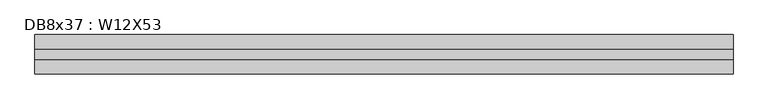
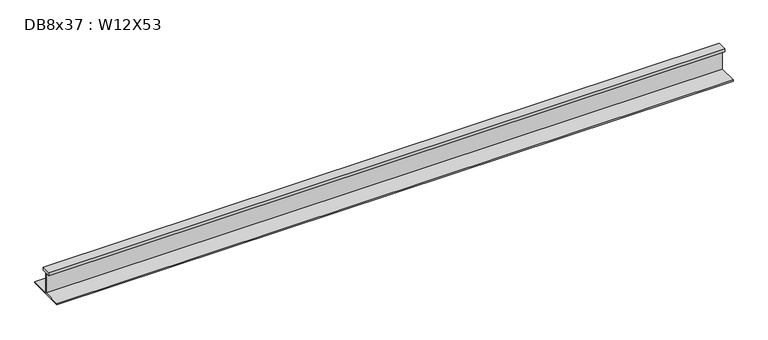
"""IFC4 building model written with IfcOpenShell, lengths in millimetres: beam geometry, DB8x37 : W12X53."""

from ifc_helpers import new_model, si_unit, frame, origin, place, context, project, spatial, polyline, outline, extrude, source, transform, mapped, element, save


def db8x37_w12x53_95cbac0b(model_context):
    return source(origin(), model_context, "Body", "SweptSolid", [
        extrude(outline(polyline([(38.1, 145.415), (38.1, 120.015), (2.921, 120.015), (2.921, -48.4505), (152.4, -48.4505), (152.4, -58.1025), (-152.4, -58.1025), (-152.4, -48.4505), (-2.921, -48.4505), (-2.921, 120.015), (-38.1, 120.015), (-38.1, 145.415), (38.1, 145.415)])), frame((-2691.1319305, 0.0, 0.0), z_axis=(1.0, 0.0, 0.0), x_axis=(0.0, 1.0, 0.0)), (0.0, 0.0, 1.0), 5387.0585186),
    ])


if __name__ == "__main__":
    model = new_model("IFC4")
    model_context = context("Model", 3, world=origin())
    ifc_project = project(units=[si_unit("LENGTHUNIT", "METRE", prefix="MILLI")], contexts=[model_context])
    site = spatial("IfcSite", under=ifc_project)
    building = spatial("IfcBuilding", under=site)
    placement = place(None, origin())
    db8x37_w12x53_shape = db8x37_w12x53_95cbac0b(model_context)
    element("IfcBeam", 1, ObjectType="DB8x37 : W12X53", at=placement, inside=building, context=model_context, shape_type="MappedRepresentation", body=[
        mapped(db8x37_w12x53_shape, transform((0.0, 0.0, 0.0), x_axis=(1.0, 0.0, 0.0), y_axis=(0.0, 1.0, 0.0), z_axis=(0.0, 0.0, 1.0))),
    ])
    save(model, "model.ifc")

# Revit data of these elements
# Type "DB8x37 : W12X53"
#   Assembly Code = "B10"
#   W = 53
#   Length [instance default] = 5' - 0"
#   bf = 0' - 10"
#   d = 1' - 0.1"
#   k = 0' - 1 3/8"
#   k2 = 0' - 0.8"
#   tf = 0' - 0.575"
#   tw = 0' - 0.345"
#   A = 0.108333 SF
#   Structural Material [instance default] = Steel ASTM A992
# Element 1 (IfcBeam, "DB8x37 : W12X53")
#   Materials on its faces: "Steel ASTM A992"
# Materials
#   "Steel ASTM A992": class "Metal", colour RGB 199 199 199, transparency 0, Description = "Structural steel 50ksi", Cost = 0
